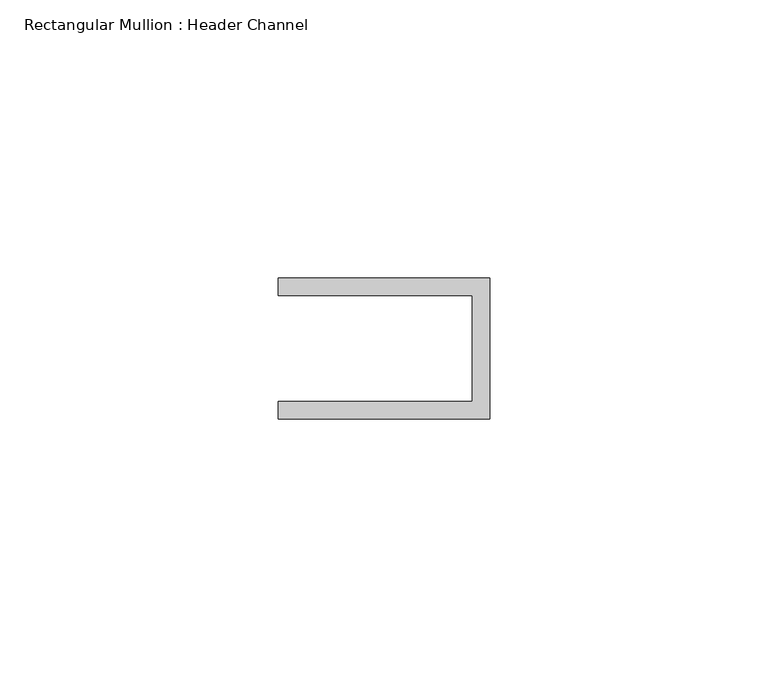
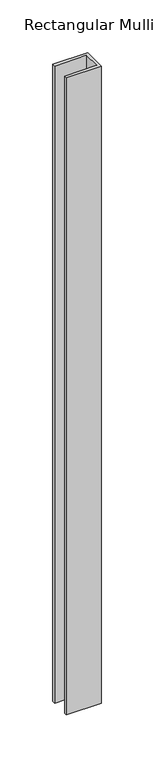
"""IFC4 building model written with IfcOpenShell, lengths in millimetres: member geometry, Rectangular Mullion : Header Channel."""

from ifc_helpers import new_model, si_unit, frame, origin, place, context, project, spatial, polyline, outline, extrude, source, transform, mapped, element, save


def rectangular_mullion_header_channel_44e32584(model_context):
    return source(origin(), model_context, "Body", "SweptSolid", [
        extrude(outline(polyline([(0.0, -12.7), (-38.1, -12.7), (-38.1, -9.525), (-3.175, -9.525), (-3.175, 9.525), (-38.1, 9.525), (-38.1, 12.7), (0.0, 12.7), (0.0, -12.7)])), frame((0.0, 0.0, -736.6), z_axis=(0.0, 0.0, 1.0), x_axis=(1.0, 0.0, 0.0)), (0.0, 0.0, 1.0), 736.6),
    ])


if __name__ == "__main__":
    model = new_model("IFC4")
    model_context = context("Model", 3, world=origin())
    ifc_project = project(units=[si_unit("LENGTHUNIT", "METRE", prefix="MILLI")], contexts=[model_context])
    site = spatial("IfcSite", under=ifc_project)
    building = spatial("IfcBuilding", under=site)
    placement = place(None, origin())
    rectangular_mullion_header_channel_shape = rectangular_mullion_header_channel_44e32584(model_context)
    element("IfcMember", 1, ObjectType="Rectangular Mullion : Header Channel", at=placement, inside=building, context=model_context, shape_type="MappedRepresentation", body=[
        mapped(rectangular_mullion_header_channel_shape, transform((0.0, 0.0, 0.0), x_axis=(1.0, 0.0, 0.0), y_axis=(0.0, 1.0, 0.0), z_axis=(0.0, 0.0, 1.0))),
    ])
    save(model, "model.ifc")

# Revit data of these elements
# Type "Rectangular Mullion : Header Channel"
#   built-in parameter 1007322 = 0.0833333 (stored number, unit not read)
#   built-in parameter 1007321 = -0.03125 (stored number, unit not read)
#   built-in parameter 1007320 = 0.0416667 (stored number, unit not read)
# Element 1 (IfcMember, "Rectangular Mullion : Header Channel")
#   Materials on its faces: "ALUM"
# Materials
#   "ALUM": class "Generic", colour RGB 157 157 157, transparency 0, Cost = 0
